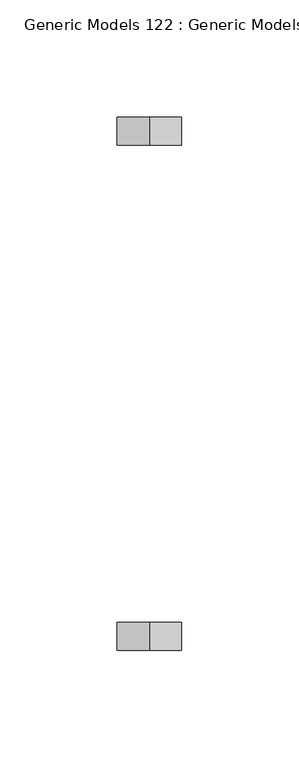
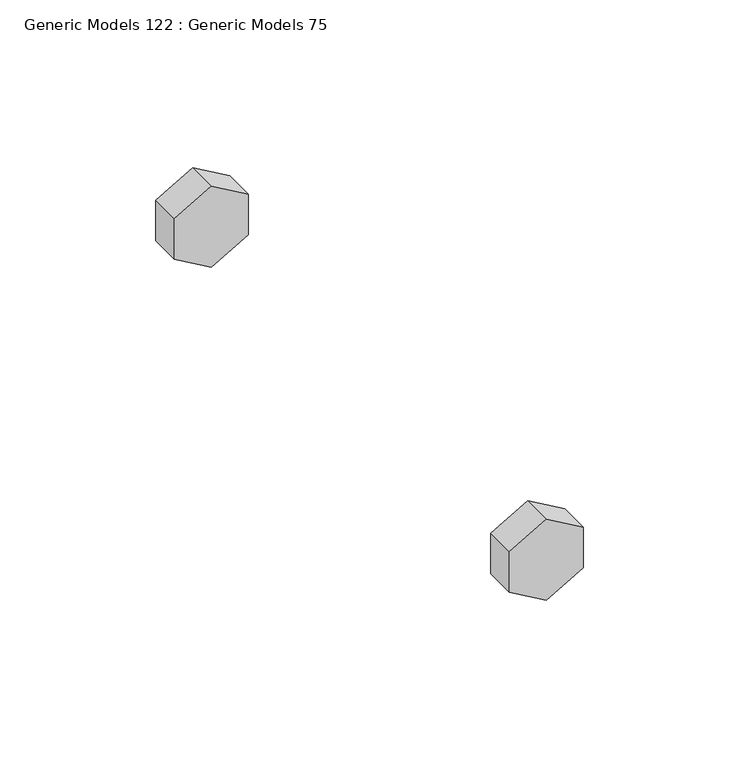
"""IFC4 building model written with IfcOpenShell, lengths in millimetres: proxy geometry, Generic Models 122 : Generic Models 75."""

from ifc_helpers import new_model, si_unit, frame, origin, place, context, project, spatial, polyline, outline, extrude, source, transform, mapped, element, save


def generic_models_122_generic_models_75_743d7a4f(model_context):
    return source(origin(), model_context, "Body", "SweptSolid", [
        extrude(outline(polyline([(269069.9462802, 31974.4067029), (269054.1097067, 31974.4067029), (269046.19142, 31988.1215778), (269054.1097067, 32001.8364528), (269069.9462802, 32001.8364528), (269077.864567, 31988.1215778), (269069.9462802, 31974.4067029)])), frame((0.0, 36509.0207942, 0.0), z_axis=(0.0, 1.0, 0.0), x_axis=(0.0, 0.0, 1.0)), (0.0, 0.0, 1.0), 11.90625),
        extrude(outline(polyline([(269069.9462802, 31974.4067029), (269054.1097067, 31974.4067029), (269046.19142, 31988.1215778), (269054.1097067, 32001.8364528), (269069.9462802, 32001.8364528), (269077.864567, 31988.1215778), (269069.9462802, 31974.4067029)])), frame((0.0, 36293.9145442, 0.0), z_axis=(0.0, 1.0, 0.0), x_axis=(0.0, 0.0, 1.0)), (0.0, 0.0, 1.0), 11.90625),
    ])


if __name__ == "__main__":
    model = new_model("IFC4")
    model_context = context("Model", 3, world=origin())
    ifc_project = project(units=[si_unit("LENGTHUNIT", "METRE", prefix="MILLI")], contexts=[model_context])
    site = spatial("IfcSite", under=ifc_project)
    building = spatial("IfcBuilding", under=site)
    placement = place(None, origin())
    generic_models_122_generic_models_75_shape = generic_models_122_generic_models_75_743d7a4f(model_context)
    element("IfcBuildingElementProxy", 1, Name="Generic Models 122 : Generic Models 75", ObjectType="Generic Models 122 : Generic Models 75", at=placement, inside=building, context=model_context, shape_type="MappedRepresentation", body=[
        mapped(generic_models_122_generic_models_75_shape, transform((0.0, 0.0, 0.0), x_axis=(1.0, 0.0, 0.0), y_axis=(0.0, 1.0, 0.0), z_axis=(0.0, 0.0, 1.0))),
    ])
    save(model, "model.ifc")

# Revit data of these elements
# Element 1 (IfcBuildingElementProxy, "Generic Models 122 : Generic Models 75")
#   Materials on its faces: "3/4\" GALV. THRU BOLTS"
# Materials
#   "3/4\" GALV. THRU BOLTS": class "Generic", colour RGB 105 69 171, transparency 0, Cost = 0
